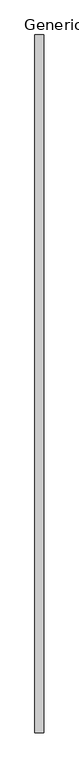
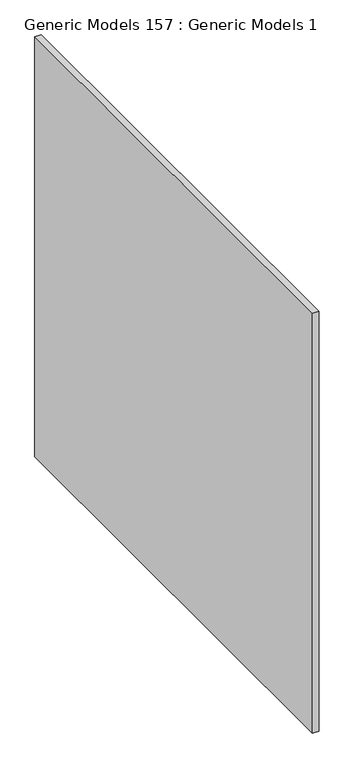
"""IFC4 building model written with IfcOpenShell, lengths in millimetres: proxy geometry, Generic Models 157 : Generic Models 1."""

import ifcopenshell
import ifcopenshell.guid

model = None  # the IFC model being written
_history = None  # IfcOwnerHistory: only IFC2X3 demands one
_inside = {}  # id of a spatial element -> (the spatial element, [elements in it])
_under = {}  # id of a project, library or spatial element -> (it, [spatial elements below it])
_declared = {}  # id of a project -> (the project, [libraries it declares])
_typed = {}  # id of a type object -> (the type object, [elements of that type])
_made_of = {}  # id of a material, layer set ... -> (it, [elements and type objects made of it])


def new_model(schema):
    """Start an empty IFC model of exactly this schema.

    Asked for "IFC4X3", IfcOpenShell would pick the latest addendum, in which some entities
    have other attributes; the version numbers below select the first issue.
    IFC2X3 requires an IfcOwnerHistory on every rooted entity: one is made here for all.
    """
    global model, _history
    if schema == "IFC4X3":
        model = ifcopenshell.file(schema_version=(4, 3, 0, 0))
    else:
        model = ifcopenshell.file(schema=schema)
    _inside.clear()
    _under.clear()
    _declared.clear()
    _typed.clear()
    _made_of.clear()
    _history = None
    if model.schema == "IFC2X3":
        org = make("IfcOrganization", Name="unknown")
        user = make(
            "IfcPersonAndOrganization",
            ThePerson=make("IfcPerson", FamilyName="unknown"),
            TheOrganization=org,
        )
        app = make(
            "IfcApplication",
            ApplicationDeveloper=org,
            Version="unknown",
            ApplicationFullName="unknown",
            ApplicationIdentifier="unknown",
        )
        _history = make(
            "IfcOwnerHistory",
            OwningUser=user,
            OwningApplication=app,
            ChangeAction="ADDED",
            CreationDate=0,
        )
    return model


def make(cls, **values):
    """One entity of the class cls with the attributes given. An attribute that is None is left unset."""
    return model.create_entity(
        cls, **{name: value for name, value in values.items() if value is not None}
    )


def rooted(cls, **values):
    """An entity with a GlobalId (a new one), such as an element, a storey or a relation."""
    return make(cls, GlobalId=ifcopenshell.guid.new(), OwnerHistory=_history, **values)


def si_unit(unit_type, name, prefix=None):
    """IfcSIUnit, for example si_unit("LENGTHUNIT", "METRE", prefix="MILLI")."""
    return make("IfcSIUnit", UnitType=unit_type, Prefix=prefix, Name=name)


def assignment(units):
    """IfcUnitAssignment: the units of a project."""
    return None if units is None else make("IfcUnitAssignment", Units=units)


def point(xyz):
    """IfcCartesianPoint."""
    return None if xyz is None else make("IfcCartesianPoint", Coordinates=xyz)


def direction(xyz):
    """IfcDirection."""
    return None if xyz is None else make("IfcDirection", DirectionRatios=xyz)


def frame(location, z_axis=None, x_axis=None):
    """IfcAxis2Placement3D, a coordinate frame: its origin and axes. An axis left out is left unset."""
    return make(
        "IfcAxis2Placement3D",
        Location=point(location),
        Axis=direction(z_axis),
        RefDirection=direction(x_axis),
    )


def origin():
    """The frame at (0, 0, 0) with its axes left unset."""
    return frame((0.0, 0.0, 0.0))


def place(relative_to, where):
    """IfcLocalPlacement: puts the frame where relative to a parent placement (None: the world)."""
    return make(
        "IfcLocalPlacement", PlacementRelTo=relative_to, RelativePlacement=where
    )


def context(
    kind, dimensions, precision=None, world=None, true_north=None, identifier=None
):
    """IfcGeometricRepresentationContext, for example the 3D "Model" context."""
    return make(
        "IfcGeometricRepresentationContext",
        ContextIdentifier=identifier,
        ContextType=kind,
        CoordinateSpaceDimension=dimensions,
        Precision=precision,
        WorldCoordinateSystem=world,
        TrueNorth=true_north,
    )


def project(units=None, contexts=None):
    """IfcProject with its units and contexts."""
    return rooted(
        "IfcProject",
        Name="project",
        RepresentationContexts=contexts,
        UnitsInContext=assignment(units),
    )


def spatial(cls, under=None, at=None, **own):
    """A site, building, storey or space (cls), placed at a placement, below another one or the project."""
    s = rooted(cls, ObjectPlacement=at, **own)
    if under is not None:
        _under.setdefault(under.id(), (under, []))[1].append(s)
    return s


def polyline(points):
    """IfcPolyline through the points."""
    return make("IfcPolyline", Points=[point(p) for p in points])


def outline(outer, holes=None, kind="AREA"):
    """IfcArbitraryClosedProfileDef: a profile drawn as a closed curve; with holes, ...WithVoids."""
    if holes is None:
        return make("IfcArbitraryClosedProfileDef", ProfileType=kind, OuterCurve=outer)
    return make(
        "IfcArbitraryProfileDefWithVoids",
        ProfileType=kind,
        OuterCurve=outer,
        InnerCurves=holes,
    )


def extrude(swept, where, along, depth):
    """IfcExtrudedAreaSolid: the profile swept, set in the frame where, extruded along a direction by depth."""
    return make(
        "IfcExtrudedAreaSolid",
        SweptArea=swept,
        Position=where,
        ExtrudedDirection=direction(along),
        Depth=depth,
    )


def shape(context_of_items, identifier, shape_type, items):
    """IfcShapeRepresentation: the items that make up one representation, for example the "Body"."""
    return make(
        "IfcShapeRepresentation",
        ContextOfItems=context_of_items,
        RepresentationIdentifier=identifier,
        RepresentationType=shape_type,
        Items=items,
    )


def source(mapping_origin, context_of_items, identifier, shape_type, items):
    """IfcRepresentationMap: a shape defined once, which mapped items show again and again."""
    return make(
        "IfcRepresentationMap",
        MappingOrigin=mapping_origin,
        MappedRepresentation=shape(context_of_items, identifier, shape_type, items),
    )


def transform(
    local_origin,
    x_axis=None,
    y_axis=None,
    z_axis=None,
    scale=None,
    scale2=None,
    scale3=None,
    uniform=True,
):
    """IfcCartesianTransformationOperator3D, or its non-uniform kind. x_axis, y_axis, z_axis: its Axis1, 2, 3."""
    if uniform:
        return make(
            "IfcCartesianTransformationOperator3D",
            Axis1=direction(x_axis),
            Axis2=direction(y_axis),
            LocalOrigin=point(local_origin),
            Scale=scale,
            Axis3=direction(z_axis),
        )
    return make(
        "IfcCartesianTransformationOperator3DnonUniform",
        Axis1=direction(x_axis),
        Axis2=direction(y_axis),
        LocalOrigin=point(local_origin),
        Scale=scale,
        Axis3=direction(z_axis),
        Scale2=scale2,
        Scale3=scale3,
    )


def mapped(mapping_source, mapping_target):
    """IfcMappedItem: shows the shape of a source again, moved by a transform."""
    return make(
        "IfcMappedItem", MappingSource=mapping_source, MappingTarget=mapping_target
    )


def made_of(thing, what):
    """Note that an element or type object is made of a material, layer set ...; save() writes the relation."""
    if what is not None:
        _made_of.setdefault(what.id(), (what, []))[1].append(thing)
    return thing


def element(
    cls,
    number,
    at=None,
    inside=None,
    cuts=None,
    type_object=None,
    material=None,
    context=None,
    identifier="Body",
    shape_type=None,
    held_by="IfcProductDefinitionShape",
    body=None,
    shapes=None,
    **own,
):
    """One element of the class cls, such as IfcWall. Its Tag is "e" and its number.

    at: its placement. inside: the storey or other place that contains it. cuts: it is an
    opening in that element (IfcRelVoidsElement). A single representation is given by context,
    identifier, shape_type and body (its items); several are given by shapes. held_by: the class
    of the entity that holds the representations. save() writes the other relations.
    """
    e = rooted(cls, Tag="e%d" % number, ObjectPlacement=at, **own)
    if body is not None:
        shapes = [shape(context, identifier, shape_type, body)]
    if shapes is not None:
        e.Representation = make(held_by, Representations=shapes)
    if inside is not None:
        _inside.setdefault(inside.id(), (inside, []))[1].append(e)
    if cuts is not None:
        rooted(
            "IfcRelVoidsElement", RelatingBuildingElement=cuts, RelatedOpeningElement=e
        )
    if type_object is not None:
        _typed.setdefault(type_object.id(), (type_object, []))[1].append(e)
    return made_of(e, material)


def aggregate(whole, parts):
    """IfcRelAggregates: a whole, such as a stair, and the parts it consists of."""
    return rooted("IfcRelAggregates", RelatingObject=whole, RelatedObjects=parts)


def save(model, path):
    """Write the relations noted so far, then the file.

    IfcRelAggregates (storeys below a building ...), IfcRelContainedInSpatialStructure (elements
    in a storey), IfcRelDefinesByType, IfcRelAssociatesMaterial and IfcRelDeclares: one each for
    every whole, place, type object, material and project.
    """
    for whole, parts in _under.values():
        aggregate(whole, parts)
    for where, things in _inside.values():
        rooted(
            "IfcRelContainedInSpatialStructure",
            RelatedElements=things,
            RelatingStructure=where,
        )
    for kind, things in _typed.values():
        rooted("IfcRelDefinesByType", RelatedObjects=things, RelatingType=kind)
    for what, things in _made_of.values():
        rooted("IfcRelAssociatesMaterial", RelatedObjects=things, RelatingMaterial=what)
    for by, libraries in _declared.values():
        rooted("IfcRelDeclares", RelatingContext=by, RelatedDefinitions=libraries)
    model.write(path)


def generic_models_157_generic_models_1_b3b9a6c0(model_context):
    return source(origin(), model_context, "Body", "SweptSolid", [
        extrude(outline(polyline([(47363.0625, 1219.2), (47363.0625, 0.0), (47347.1875, 0.0), (47347.1875, 1219.2), (47363.0625, 1219.2)])), frame((0.0, 0.0, 4267.2), z_axis=(0.0, 0.0, 1.0), x_axis=(1.0, 0.0, 0.0)), (0.0, 0.0, 1.0), 1123.95),
    ])


if __name__ == "__main__":
    model = new_model("IFC4")
    model_context = context("Model", 3, world=origin())
    ifc_project = project(units=[si_unit("LENGTHUNIT", "METRE", prefix="MILLI")], contexts=[model_context])
    site = spatial("IfcSite", under=ifc_project)
    building = spatial("IfcBuilding", under=site)
    placement = place(None, origin())
    generic_models_157_generic_models_1_shape = generic_models_157_generic_models_1_b3b9a6c0(model_context)
    element("IfcBuildingElementProxy", 1, Name="Generic Models 157 : Generic Models 1", ObjectType="Generic Models 157 : Generic Models 1", at=placement, inside=building, context=model_context, shape_type="MappedRepresentation", body=[
        mapped(generic_models_157_generic_models_1_shape, transform((0.0, 0.0, 0.0), x_axis=(1.0, 0.0, 0.0), y_axis=(0.0, 1.0, 0.0), z_axis=(0.0, 0.0, 1.0))),
    ])
    save(model, "model.ifc")

# Revit data of these elements
# Element 1 (IfcBuildingElementProxy, "Generic Models 157 : Generic Models 1")
#   Materials on its faces: "GYP. BD (SEE 'WALL TAG' & 'LAYER MATERIAL SCHEDULE' FOR DETAILS)"
# Materials
#   "GYP. BD (SEE 'WALL TAG' & 'LAYER MATERIAL SCHEDULE' FOR DETAILS)": class "Generic", colour RGB 237 236 233, transparency 0, Description = "Gypsum Wall Board", Cost = 0
